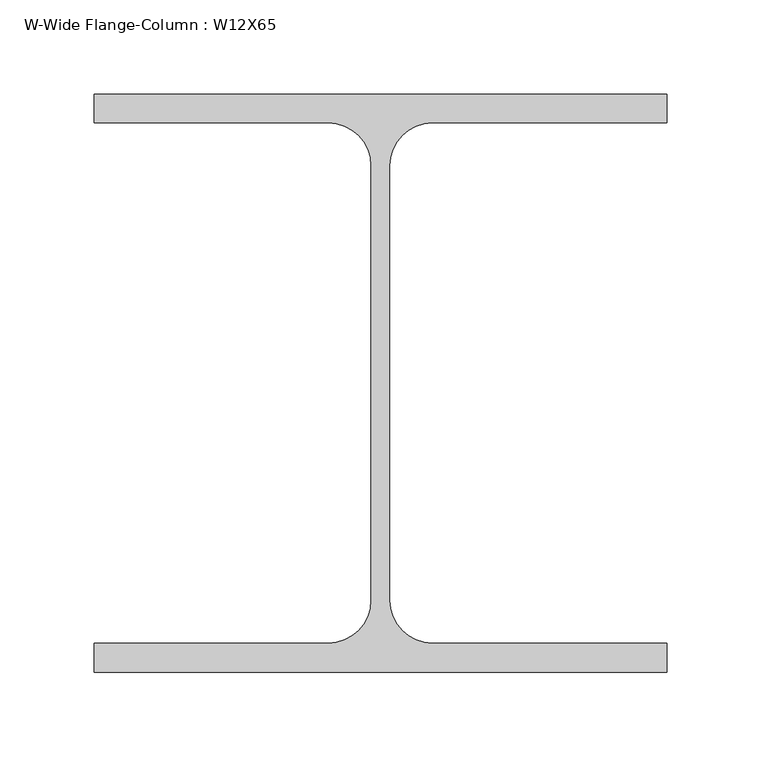
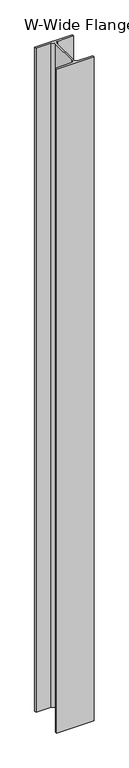
"""IFC4 building model written with IfcOpenShell, lengths in millimetres: column geometry, W-Wide Flange-Column : W12X65."""

from ifc_helpers import new_model, si_unit, point, frame, frame_2d, origin, place, context, project, spatial, polyline, circle_curve, trimmed, segment, composite_curve, outline, extrude, source, transform, mapped, element, save


def w_wide_flange_column_w12x65_26eae5e9(model_context):
    return source(origin(), model_context, "Body", "SweptSolid", [
        extrude(outline(composite_curve([segment(polyline([(152.4, 153.67), (152.4, 138.303), (27.686, 138.303)]), True, "CONTINUOUS"), segment(trimmed(circle_curve(frame_2d((27.686, 115.57)), 22.733), [point((27.686, 138.303))], [point((4.953, 115.57))], True, "CARTESIAN"), True, "CONTINUOUS"), segment(polyline([(4.953, 115.57), (4.953, -115.57)]), True, "CONTINUOUS"), segment(trimmed(circle_curve(frame_2d((27.686, -115.57)), 22.733), [point((4.953, -115.57))], [point((27.686, -138.303))], True, "CARTESIAN"), True, "CONTINUOUS"), segment(polyline([(27.686, -138.303), (152.4, -138.303), (152.4, -153.67), (-152.4, -153.67), (-152.4, -138.303), (-27.686, -138.303)]), True, "CONTINUOUS"), segment(trimmed(circle_curve(frame_2d((-27.686, -115.57)), 22.733), [point((-27.686, -138.303))], [point((-4.953, -115.57))], True, "CARTESIAN"), True, "CONTINUOUS"), segment(polyline([(-4.953, -115.57), (-4.953, 115.57)]), True, "CONTINUOUS"), segment(trimmed(circle_curve(frame_2d((-27.686, 115.57)), 22.733), [point((-4.953, 115.57))], [point((-27.686, 138.303))], True, "CARTESIAN"), True, "CONTINUOUS"), segment(polyline([(-27.686, 138.303), (-152.4, 138.303), (-152.4, 153.67), (152.4, 153.67)]), True, "CONTINUOUS")], self_intersect=False)), frame((0.0, 0.0, 17627.6), z_axis=(0.0, 0.0, 1.0), x_axis=(1.0, 0.0, 0.0)), (0.0, 0.0, 1.0), 5689.6),
    ])


if __name__ == "__main__":
    model = new_model("IFC4")
    model_context = context("Model", 3, world=origin())
    ifc_project = project(units=[si_unit("LENGTHUNIT", "METRE", prefix="MILLI")], contexts=[model_context])
    site = spatial("IfcSite", under=ifc_project)
    building = spatial("IfcBuilding", under=site)
    placement = place(None, origin())
    w_wide_flange_column_w12x65_shape = w_wide_flange_column_w12x65_26eae5e9(model_context)
    element("IfcColumn", 1, ObjectType="W-Wide Flange-Column : W12X65", at=placement, inside=building, context=model_context, shape_type="MappedRepresentation", body=[
        mapped(w_wide_flange_column_w12x65_shape, transform((0.0, 0.0, 0.0), x_axis=(1.0, 0.0, 0.0), y_axis=(0.0, 1.0, 0.0), z_axis=(0.0, 0.0, 1.0))),
    ])
    save(model, "model.ifc")

# Revit data of these elements
# Type "W-Wide Flange-Column : W12X65"
#   Assembly Code = "B10"
#   W = 65
#   bf = 1' - 0"
#   d = 1' - 0.1"
#   k = 0' - 1 1/2"
#   kr = 0' - 0.895"
#   tf = 0' - 0.605"
#   tw = 0' - 0.39"
#   A = 0.132639 SF
#   Structural Material [instance default] = Steel ASTM A992
# Element 1 (IfcColumn, "W-Wide Flange-Column : W12X65")
#   Materials on its faces: "Steel ASTM A992"
# Materials
#   "Steel ASTM A992": class "Metal", colour RGB 199 199 199, transparency 0, Description = "Structural steel 50ksi", Cost = 0
